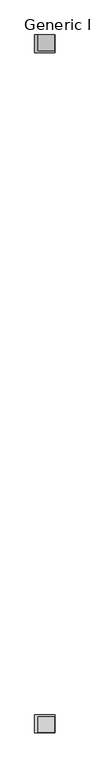
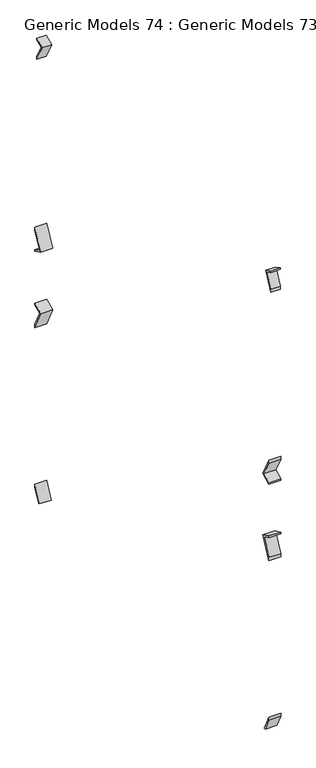
"""IFC4 building model written with IfcOpenShell, lengths in millimetres: proxy geometry, Generic Models 74 : Generic Models 73."""

from ifc_helpers import new_model, si_unit, frame, origin, place, context, project, spatial, polyline, outline, extrude, source, transform, mapped, element, save


def generic_models_74_generic_models_73_30af4f77(model_context):
    return source(origin(), model_context, "Body", "SweptSolid", [
        extrude(outline(polyline([(35205.6832942, 269257.8807194), (35205.6832942, 269240.0084236), (35094.4546362, 269297.5317044), (35205.6832942, 269512.606613), (35205.6832942, 269478.0482316), (35115.8480059, 269304.3401536), (35205.6832942, 269257.8807194)])), frame((31926.2090778, 0.0, 0.0), z_axis=(1.0, 0.0, 0.0), x_axis=(0.0, 1.0, 0.0)), (0.0, 0.0, 1.0), 127.0),
        extrude(outline(polyline([(35096.1491672, 268599.5368539), (35205.6832942, 268652.9589106), (35205.6832942, 268635.2964378), (35117.3765942, 268592.2274358), (35205.6832942, 268411.1674413), (35205.6832942, 268374.9531198), (35096.1491672, 268599.5368539)])), frame((31926.2090778, 0.0, 0.0), z_axis=(1.0, 0.0, 0.0), x_axis=(0.0, 1.0, 0.0)), (0.0, 0.0, 1.0), 127.0),
        extrude(outline(polyline([(30858.4781612, 268653.1048878), (30968.5126148, 268599.284017), (30858.4781612, 268374.323313), (30858.4781612, 268410.4535164), (30947.2768993, 268591.9987142), (30858.4781612, 268635.4326138), (30858.4781612, 268653.1048878)])), frame((31926.2090778, 0.0, 0.0), z_axis=(1.0, 0.0, 0.0), x_axis=(0.0, 1.0, 0.0)), (0.0, 0.0, 1.0), 127.0),
        extrude(outline(polyline([(30858.4781612, 269511.403569), (30969.8193559, 269297.6283572), (30858.4781612, 269239.6381837), (30858.4781612, 269257.5373223), (30948.4063874, 269304.3749142), (30858.4781612, 269477.0372039), (30858.4781612, 269511.403569)])), frame((31926.2090778, 0.0, 0.0), z_axis=(1.0, 0.0, 0.0), x_axis=(0.0, 1.0, 0.0)), (0.0, 0.0, 1.0), 127.0),
        extrude(outline(polyline([(30858.4781612, 266604.159959), (30945.7795167, 266422.1875), (30929.2647163, 266422.1875), (30858.4781612, 266567.3214459), (30858.4781612, 266604.159959)])), frame((31926.2090778, 0.0, 0.0), z_axis=(1.0, 0.0, 0.0), x_axis=(0.0, 1.0, 0.0)), (0.0, 0.0, 1.0), 127.0),
        extrude(outline(polyline([(35121.9487208, 266430.125), (35205.6832942, 266604.159959), (35205.6832942, 266567.5560345), (35138.4620039, 266430.125), (35121.9487208, 266430.125)])), frame((31926.2090778, 0.0, 0.0), z_axis=(1.0, 0.0, 0.0), x_axis=(0.0, 1.0, 0.0)), (0.0, 0.0, 1.0), 127.0),
        extrude(outline(polyline([(35107.5372238, 271593.3298996), (35205.6832942, 271644.1006278), (35205.6832942, 271626.2273459), (35128.9313197, 271586.5237325), (35205.6832942, 271438.1527132), (35205.6832942, 271403.6014581), (35107.5372238, 271593.3298996)])), frame((31948.4340778, 0.0, 0.0), z_axis=(1.0, 0.0, 0.0), x_axis=(0.0, 1.0, 0.0)), (0.0, 0.0, 1.0), 101.6),
        extrude(outline(polyline([(30956.6242316, 271593.3298996), (30858.4781612, 271403.6014581), (30858.4781612, 271438.1527132), (30935.2301357, 271586.5237325), (30858.4781612, 271626.2273459), (30858.4781612, 271644.1006278), (30956.6242316, 271593.3298996)])), frame((31948.4340778, 0.0, 0.0), z_axis=(1.0, 0.0, 0.0), x_axis=(0.0, 1.0, 0.0)), (0.0, 0.0, 1.0), 101.6),
    ])


if __name__ == "__main__":
    model = new_model("IFC4")
    model_context = context("Model", 3, world=origin())
    ifc_project = project(units=[si_unit("LENGTHUNIT", "METRE", prefix="MILLI")], contexts=[model_context])
    site = spatial("IfcSite", under=ifc_project)
    building = spatial("IfcBuilding", under=site)
    placement = place(None, origin())
    generic_models_74_generic_models_73_shape = generic_models_74_generic_models_73_30af4f77(model_context)
    element("IfcBuildingElementProxy", 1, Name="Generic Models 74 : Generic Models 73", ObjectType="Generic Models 74 : Generic Models 73", at=placement, inside=building, context=model_context, shape_type="MappedRepresentation", body=[
        mapped(generic_models_74_generic_models_73_shape, transform((0.0, 0.0, 0.0), x_axis=(1.0, 0.0, 0.0), y_axis=(0.0, 1.0, 0.0), z_axis=(0.0, 0.0, 1.0))),
    ])
    save(model, "model.ifc")

# Revit data of these elements
# Element 1 (IfcBuildingElementProxy, "Generic Models 74 : Generic Models 73")
#   Materials on its faces: "5/8\" BENT PLATE, FIELD WELD - PAINT WELDS WITH ZINC RICH PAINT TO MATCH GALV. FINISH"
# Materials
#   "5/8\" BENT PLATE, FIELD WELD - PAINT WELDS WITH ZINC RICH PAINT TO MATCH GALV. FINISH": class "Metal", colour RGB 199 199 199, transparency 0, Description = "Carbon steel", Cost = 0
